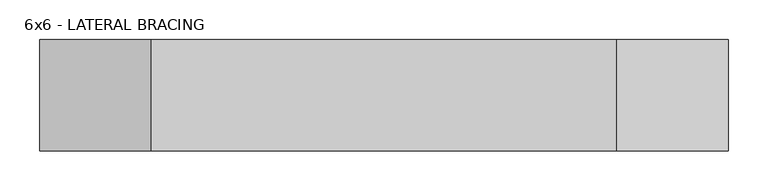
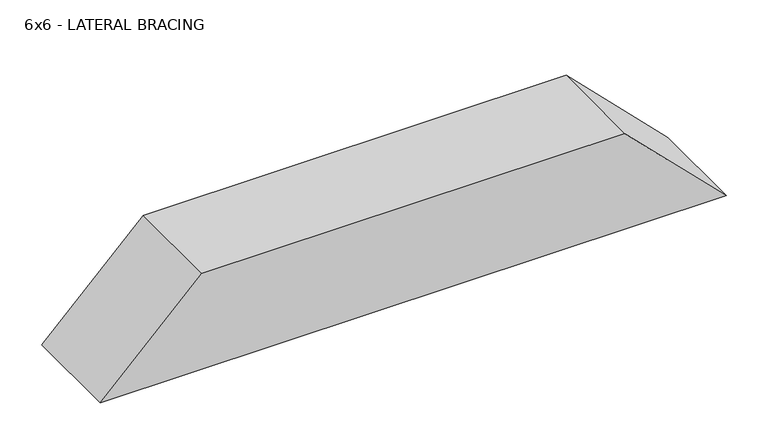
"""IFC4 building model written with IfcOpenShell, lengths in millimetres: member geometry, Dimension Lumber - Canted Ends : 6x6 - LATERAL BRACING."""

import ifcopenshell
import ifcopenshell.guid

model = None  # the IFC model being written
_history = None  # IfcOwnerHistory: only IFC2X3 demands one
_inside = {}  # id of a spatial element -> (the spatial element, [elements in it])
_under = {}  # id of a project, library or spatial element -> (it, [spatial elements below it])
_declared = {}  # id of a project -> (the project, [libraries it declares])
_typed = {}  # id of a type object -> (the type object, [elements of that type])
_made_of = {}  # id of a material, layer set ... -> (it, [elements and type objects made of it])


def new_model(schema):
    """Start an empty IFC model of exactly this schema.

    Asked for "IFC4X3", IfcOpenShell would pick the latest addendum, in which some entities
    have other attributes; the version numbers below select the first issue.
    IFC2X3 requires an IfcOwnerHistory on every rooted entity: one is made here for all.
    """
    global model, _history
    if schema == "IFC4X3":
        model = ifcopenshell.file(schema_version=(4, 3, 0, 0))
    else:
        model = ifcopenshell.file(schema=schema)
    _inside.clear()
    _under.clear()
    _declared.clear()
    _typed.clear()
    _made_of.clear()
    _history = None
    if model.schema == "IFC2X3":
        org = make("IfcOrganization", Name="unknown")
        user = make(
            "IfcPersonAndOrganization",
            ThePerson=make("IfcPerson", FamilyName="unknown"),
            TheOrganization=org,
        )
        app = make(
            "IfcApplication",
            ApplicationDeveloper=org,
            Version="unknown",
            ApplicationFullName="unknown",
            ApplicationIdentifier="unknown",
        )
        _history = make(
            "IfcOwnerHistory",
            OwningUser=user,
            OwningApplication=app,
            ChangeAction="ADDED",
            CreationDate=0,
        )
    return model


def make(cls, **values):
    """One entity of the class cls with the attributes given. An attribute that is None is left unset."""
    return model.create_entity(
        cls, **{name: value for name, value in values.items() if value is not None}
    )


def rooted(cls, **values):
    """An entity with a GlobalId (a new one), such as an element, a storey or a relation."""
    return make(cls, GlobalId=ifcopenshell.guid.new(), OwnerHistory=_history, **values)


def si_unit(unit_type, name, prefix=None):
    """IfcSIUnit, for example si_unit("LENGTHUNIT", "METRE", prefix="MILLI")."""
    return make("IfcSIUnit", UnitType=unit_type, Prefix=prefix, Name=name)


def assignment(units):
    """IfcUnitAssignment: the units of a project."""
    return None if units is None else make("IfcUnitAssignment", Units=units)


def point(xyz):
    """IfcCartesianPoint."""
    return None if xyz is None else make("IfcCartesianPoint", Coordinates=xyz)


def direction(xyz):
    """IfcDirection."""
    return None if xyz is None else make("IfcDirection", DirectionRatios=xyz)


def frame(location, z_axis=None, x_axis=None):
    """IfcAxis2Placement3D, a coordinate frame: its origin and axes. An axis left out is left unset."""
    return make(
        "IfcAxis2Placement3D",
        Location=point(location),
        Axis=direction(z_axis),
        RefDirection=direction(x_axis),
    )


def origin():
    """The frame at (0, 0, 0) with its axes left unset."""
    return frame((0.0, 0.0, 0.0))


def place(relative_to, where):
    """IfcLocalPlacement: puts the frame where relative to a parent placement (None: the world)."""
    return make(
        "IfcLocalPlacement", PlacementRelTo=relative_to, RelativePlacement=where
    )


def context(
    kind, dimensions, precision=None, world=None, true_north=None, identifier=None
):
    """IfcGeometricRepresentationContext, for example the 3D "Model" context."""
    return make(
        "IfcGeometricRepresentationContext",
        ContextIdentifier=identifier,
        ContextType=kind,
        CoordinateSpaceDimension=dimensions,
        Precision=precision,
        WorldCoordinateSystem=world,
        TrueNorth=true_north,
    )


def project(units=None, contexts=None):
    """IfcProject with its units and contexts."""
    return rooted(
        "IfcProject",
        Name="project",
        RepresentationContexts=contexts,
        UnitsInContext=assignment(units),
    )


def spatial(cls, under=None, at=None, **own):
    """A site, building, storey or space (cls), placed at a placement, below another one or the project."""
    s = rooted(cls, ObjectPlacement=at, **own)
    if under is not None:
        _under.setdefault(under.id(), (under, []))[1].append(s)
    return s


def polyline(points):
    """IfcPolyline through the points."""
    return make("IfcPolyline", Points=[point(p) for p in points])


def outline(outer, holes=None, kind="AREA"):
    """IfcArbitraryClosedProfileDef: a profile drawn as a closed curve; with holes, ...WithVoids."""
    if holes is None:
        return make("IfcArbitraryClosedProfileDef", ProfileType=kind, OuterCurve=outer)
    return make(
        "IfcArbitraryProfileDefWithVoids",
        ProfileType=kind,
        OuterCurve=outer,
        InnerCurves=holes,
    )


def extrude(swept, where, along, depth):
    """IfcExtrudedAreaSolid: the profile swept, set in the frame where, extruded along a direction by depth."""
    return make(
        "IfcExtrudedAreaSolid",
        SweptArea=swept,
        Position=where,
        ExtrudedDirection=direction(along),
        Depth=depth,
    )


def shape(context_of_items, identifier, shape_type, items):
    """IfcShapeRepresentation: the items that make up one representation, for example the "Body"."""
    return make(
        "IfcShapeRepresentation",
        ContextOfItems=context_of_items,
        RepresentationIdentifier=identifier,
        RepresentationType=shape_type,
        Items=items,
    )


def source(mapping_origin, context_of_items, identifier, shape_type, items):
    """IfcRepresentationMap: a shape defined once, which mapped items show again and again."""
    return make(
        "IfcRepresentationMap",
        MappingOrigin=mapping_origin,
        MappedRepresentation=shape(context_of_items, identifier, shape_type, items),
    )


def transform(
    local_origin,
    x_axis=None,
    y_axis=None,
    z_axis=None,
    scale=None,
    scale2=None,
    scale3=None,
    uniform=True,
):
    """IfcCartesianTransformationOperator3D, or its non-uniform kind. x_axis, y_axis, z_axis: its Axis1, 2, 3."""
    if uniform:
        return make(
            "IfcCartesianTransformationOperator3D",
            Axis1=direction(x_axis),
            Axis2=direction(y_axis),
            LocalOrigin=point(local_origin),
            Scale=scale,
            Axis3=direction(z_axis),
        )
    return make(
        "IfcCartesianTransformationOperator3DnonUniform",
        Axis1=direction(x_axis),
        Axis2=direction(y_axis),
        LocalOrigin=point(local_origin),
        Scale=scale,
        Axis3=direction(z_axis),
        Scale2=scale2,
        Scale3=scale3,
    )


def mapped(mapping_source, mapping_target):
    """IfcMappedItem: shows the shape of a source again, moved by a transform."""
    return make(
        "IfcMappedItem", MappingSource=mapping_source, MappingTarget=mapping_target
    )


def made_of(thing, what):
    """Note that an element or type object is made of a material, layer set ...; save() writes the relation."""
    if what is not None:
        _made_of.setdefault(what.id(), (what, []))[1].append(thing)
    return thing


def element(
    cls,
    number,
    at=None,
    inside=None,
    cuts=None,
    type_object=None,
    material=None,
    context=None,
    identifier="Body",
    shape_type=None,
    held_by="IfcProductDefinitionShape",
    body=None,
    shapes=None,
    **own,
):
    """One element of the class cls, such as IfcWall. Its Tag is "e" and its number.

    at: its placement. inside: the storey or other place that contains it. cuts: it is an
    opening in that element (IfcRelVoidsElement). A single representation is given by context,
    identifier, shape_type and body (its items); several are given by shapes. held_by: the class
    of the entity that holds the representations. save() writes the other relations.
    """
    e = rooted(cls, Tag="e%d" % number, ObjectPlacement=at, **own)
    if body is not None:
        shapes = [shape(context, identifier, shape_type, body)]
    if shapes is not None:
        e.Representation = make(held_by, Representations=shapes)
    if inside is not None:
        _inside.setdefault(inside.id(), (inside, []))[1].append(e)
    if cuts is not None:
        rooted(
            "IfcRelVoidsElement", RelatingBuildingElement=cuts, RelatedOpeningElement=e
        )
    if type_object is not None:
        _typed.setdefault(type_object.id(), (type_object, []))[1].append(e)
    return made_of(e, material)


def aggregate(whole, parts):
    """IfcRelAggregates: a whole, such as a stair, and the parts it consists of."""
    return rooted("IfcRelAggregates", RelatingObject=whole, RelatedObjects=parts)


def save(model, path):
    """Write the relations noted so far, then the file.

    IfcRelAggregates (storeys below a building ...), IfcRelContainedInSpatialStructure (elements
    in a storey), IfcRelDefinesByType, IfcRelAssociatesMaterial and IfcRelDeclares: one each for
    every whole, place, type object, material and project.
    """
    for whole, parts in _under.values():
        aggregate(whole, parts)
    for where, things in _inside.values():
        rooted(
            "IfcRelContainedInSpatialStructure",
            RelatedElements=things,
            RelatingStructure=where,
        )
    for kind, things in _typed.values():
        rooted("IfcRelDefinesByType", RelatedObjects=things, RelatingType=kind)
    for what, things in _made_of.values():
        rooted("IfcRelAssociatesMaterial", RelatedObjects=things, RelatingMaterial=what)
    for by, libraries in _declared.values():
        rooted("IfcRelDeclares", RelatingContext=by, RelatedDefinitions=libraries)
    model.write(path)


def member_6x6_lateral_bracing_aa796058(model_context):
    return source(origin(), model_context, "Body", "SweptSolid", [
        extrude(outline(polyline([(-69.85, -430.9872), (-69.85, 430.9872), (69.85, 291.2872), (69.85, -291.2872), (-69.85, -430.9872)])), frame((0.0, -69.85, 0.0), z_axis=(0.0, 1.0, 0.0), x_axis=(0.0, 0.0, 1.0)), (0.0, 0.0, 1.0), 139.7),
    ])


if __name__ == "__main__":
    model = new_model("IFC4")
    model_context = context("Model", 3, world=origin())
    ifc_project = project(units=[si_unit("LENGTHUNIT", "METRE", prefix="MILLI")], contexts=[model_context])
    site = spatial("IfcSite", under=ifc_project)
    building = spatial("IfcBuilding", under=site)
    placement = place(None, origin())
    member_6x6_lateral_bracing_shape = member_6x6_lateral_bracing_aa796058(model_context)
    element("IfcMember", 1, ObjectType="Dimension Lumber - Canted Ends : 6x6 - LATERAL BRACING", at=placement, inside=building, context=model_context, shape_type="MappedRepresentation", body=[
        mapped(member_6x6_lateral_bracing_shape, transform((0.0, 0.0, 0.0), x_axis=(1.0, 0.0, 0.0), y_axis=(0.0, 1.0, 0.0), z_axis=(0.0, 0.0, 1.0))),
    ])
    save(model, "model.ifc")

# Revit data of these elements
# Type "Dimension Lumber - Canted Ends : 6x6 - LATERAL BRACING"
#   Assembly Code = "B10"
#   Angle_End = 45.00°
#   Angle_Start = 45.00°
#   A = 0.0963889 SF
#   Length [instance default] = 5' - 0"
#   b = 0' - 5 1/2"
#   d = 0' - 5 1/2"
#   Structural Material = 6X6 TREATED LATERAL BRACE
# Element 1 (IfcMember, "Dimension Lumber - Canted Ends : 6x6 - LATERAL BRACING")
#   Materials on its faces: "6X6 TREATED LATERAL BRACE"
# Materials
#   "6X6 TREATED LATERAL BRACE": class "Wood", colour RGB 234 198 147, transparency 0, Description = "Pinus Echinata", Cost = 0
